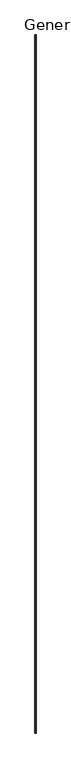
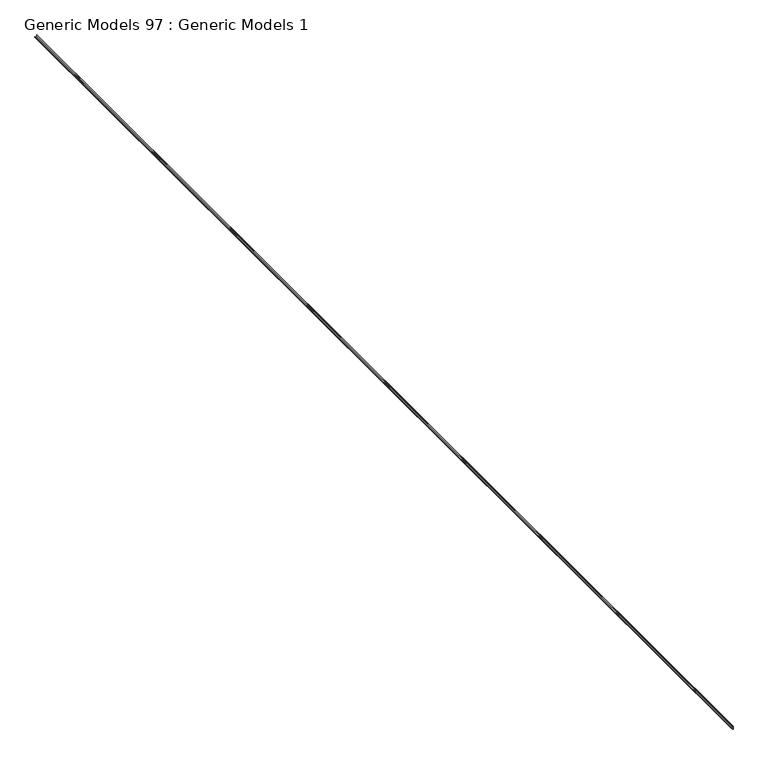
"""IFC4 building model written with IfcOpenShell, lengths in millimetres: proxy geometry, Generic Models 97 : Generic Models 1."""

from ifc_helpers import new_model, si_unit, frame, origin, place, context, project, spatial, polyline, outline, extrude, source, transform, mapped, element, save


def generic_models_97_generic_models_1_f131ade9(model_context):
    return source(origin(), model_context, "Body", "SweptSolid", [
        extrude(outline(polyline([(126669.546, -8872.7331401), (126708.916, -8872.7331401), (126708.916, -8874.0031401), (126689.866, -8874.0031401), (126689.866, -8893.6881401), (126693.3458, -8893.6881401), (126693.3458, -8894.9581401), (126688.596, -8894.9581401), (126688.596, -8874.0031401), (126669.546, -8874.0031401), (126669.546, -8872.7331401)])), frame((0.0, -7068.1230338, 0.0), z_axis=(0.0, 1.0, 0.0), x_axis=(0.0, 0.0, 1.0)), (0.0, 0.0, 1.0), 14122.4),
    ])


if __name__ == "__main__":
    model = new_model("IFC4")
    model_context = context("Model", 3, world=origin())
    ifc_project = project(units=[si_unit("LENGTHUNIT", "METRE", prefix="MILLI")], contexts=[model_context])
    site = spatial("IfcSite", under=ifc_project)
    building = spatial("IfcBuilding", under=site)
    placement = place(None, origin())
    generic_models_97_generic_models_1_shape = generic_models_97_generic_models_1_f131ade9(model_context)
    element("IfcBuildingElementProxy", 1, Name="Generic Models 97 : Generic Models 1", ObjectType="Generic Models 97 : Generic Models 1", at=placement, inside=building, context=model_context, shape_type="MappedRepresentation", body=[
        mapped(generic_models_97_generic_models_1_shape, transform((0.0, 0.0, 0.0), x_axis=(1.0, 0.0, 0.0), y_axis=(0.0, 1.0, 0.0), z_axis=(0.0, 0.0, 1.0))),
    ])
    save(model, "model.ifc")

# Revit data of these elements
# Element 1 (IfcBuildingElementProxy, "Generic Models 97 : Generic Models 1")
#   Materials on its faces: "_ 16 GA. COPPER VENTED T REVEAL BEAD (CONT. AROUND PERIMETER OF BEAM)"
# Materials
#   "_ 16 GA. COPPER VENTED T REVEAL BEAD (CONT. AROUND PERIMETER OF BEAM)": class "Generic", colour RGB 253 192 103, transparency 0, Cost = 0
